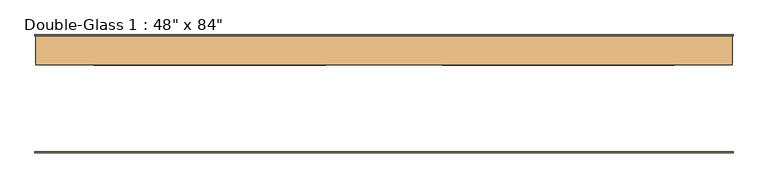
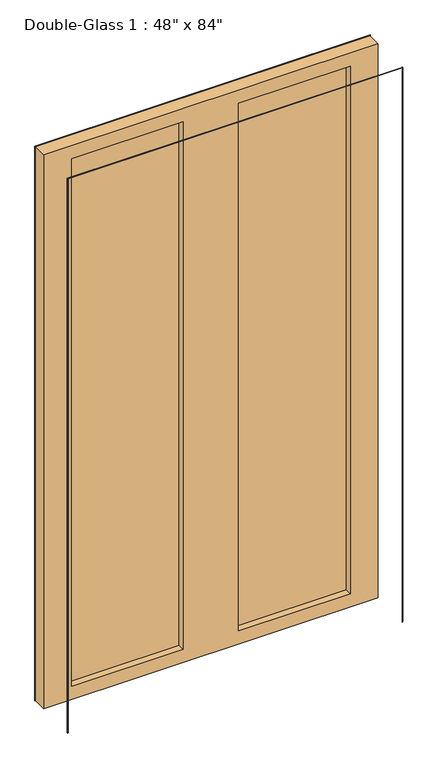
"""IFC4 building model written with IfcOpenShell, lengths in millimetres: door geometry."""

import ifcopenshell
import ifcopenshell.guid

model = None  # the IFC model being written
_history = None  # IfcOwnerHistory: only IFC2X3 demands one
_inside = {}  # id of a spatial element -> (the spatial element, [elements in it])
_under = {}  # id of a project, library or spatial element -> (it, [spatial elements below it])
_declared = {}  # id of a project -> (the project, [libraries it declares])
_typed = {}  # id of a type object -> (the type object, [elements of that type])
_made_of = {}  # id of a material, layer set ... -> (it, [elements and type objects made of it])


def new_model(schema):
    """Start an empty IFC model of exactly this schema.

    Asked for "IFC4X3", IfcOpenShell would pick the latest addendum, in which some entities
    have other attributes; the version numbers below select the first issue.
    IFC2X3 requires an IfcOwnerHistory on every rooted entity: one is made here for all.
    """
    global model, _history
    if schema == "IFC4X3":
        model = ifcopenshell.file(schema_version=(4, 3, 0, 0))
    else:
        model = ifcopenshell.file(schema=schema)
    _inside.clear()
    _under.clear()
    _declared.clear()
    _typed.clear()
    _made_of.clear()
    _history = None
    if model.schema == "IFC2X3":
        org = make("IfcOrganization", Name="unknown")
        user = make(
            "IfcPersonAndOrganization",
            ThePerson=make("IfcPerson", FamilyName="unknown"),
            TheOrganization=org,
        )
        app = make(
            "IfcApplication",
            ApplicationDeveloper=org,
            Version="unknown",
            ApplicationFullName="unknown",
            ApplicationIdentifier="unknown",
        )
        _history = make(
            "IfcOwnerHistory",
            OwningUser=user,
            OwningApplication=app,
            ChangeAction="ADDED",
            CreationDate=0,
        )
    return model


def make(cls, **values):
    """One entity of the class cls with the attributes given. An attribute that is None is left unset."""
    return model.create_entity(
        cls, **{name: value for name, value in values.items() if value is not None}
    )


def rooted(cls, **values):
    """An entity with a GlobalId (a new one), such as an element, a storey or a relation."""
    return make(cls, GlobalId=ifcopenshell.guid.new(), OwnerHistory=_history, **values)


def si_unit(unit_type, name, prefix=None):
    """IfcSIUnit, for example si_unit("LENGTHUNIT", "METRE", prefix="MILLI")."""
    return make("IfcSIUnit", UnitType=unit_type, Prefix=prefix, Name=name)


def assignment(units):
    """IfcUnitAssignment: the units of a project."""
    return None if units is None else make("IfcUnitAssignment", Units=units)


def point(xyz):
    """IfcCartesianPoint."""
    return None if xyz is None else make("IfcCartesianPoint", Coordinates=xyz)


def direction(xyz):
    """IfcDirection."""
    return None if xyz is None else make("IfcDirection", DirectionRatios=xyz)


def frame(location, z_axis=None, x_axis=None):
    """IfcAxis2Placement3D, a coordinate frame: its origin and axes. An axis left out is left unset."""
    return make(
        "IfcAxis2Placement3D",
        Location=point(location),
        Axis=direction(z_axis),
        RefDirection=direction(x_axis),
    )


def origin():
    """The frame at (0, 0, 0) with its axes left unset."""
    return frame((0.0, 0.0, 0.0))


def place(relative_to, where):
    """IfcLocalPlacement: puts the frame where relative to a parent placement (None: the world)."""
    return make(
        "IfcLocalPlacement", PlacementRelTo=relative_to, RelativePlacement=where
    )


def context(
    kind, dimensions, precision=None, world=None, true_north=None, identifier=None
):
    """IfcGeometricRepresentationContext, for example the 3D "Model" context."""
    return make(
        "IfcGeometricRepresentationContext",
        ContextIdentifier=identifier,
        ContextType=kind,
        CoordinateSpaceDimension=dimensions,
        Precision=precision,
        WorldCoordinateSystem=world,
        TrueNorth=true_north,
    )


def project(units=None, contexts=None):
    """IfcProject with its units and contexts."""
    return rooted(
        "IfcProject",
        Name="project",
        RepresentationContexts=contexts,
        UnitsInContext=assignment(units),
    )


def spatial(cls, under=None, at=None, **own):
    """A site, building, storey or space (cls), placed at a placement, below another one or the project."""
    s = rooted(cls, ObjectPlacement=at, **own)
    if under is not None:
        _under.setdefault(under.id(), (under, []))[1].append(s)
    return s


def polyline(points):
    """IfcPolyline through the points."""
    return make("IfcPolyline", Points=[point(p) for p in points])


def outline(outer, holes=None, kind="AREA"):
    """IfcArbitraryClosedProfileDef: a profile drawn as a closed curve; with holes, ...WithVoids."""
    if holes is None:
        return make("IfcArbitraryClosedProfileDef", ProfileType=kind, OuterCurve=outer)
    return make(
        "IfcArbitraryProfileDefWithVoids",
        ProfileType=kind,
        OuterCurve=outer,
        InnerCurves=holes,
    )


def extrude(swept, where, along, depth):
    """IfcExtrudedAreaSolid: the profile swept, set in the frame where, extruded along a direction by depth."""
    return make(
        "IfcExtrudedAreaSolid",
        SweptArea=swept,
        Position=where,
        ExtrudedDirection=direction(along),
        Depth=depth,
    )


def shape(context_of_items, identifier, shape_type, items):
    """IfcShapeRepresentation: the items that make up one representation, for example the "Body"."""
    return make(
        "IfcShapeRepresentation",
        ContextOfItems=context_of_items,
        RepresentationIdentifier=identifier,
        RepresentationType=shape_type,
        Items=items,
    )


def source(mapping_origin, context_of_items, identifier, shape_type, items):
    """IfcRepresentationMap: a shape defined once, which mapped items show again and again."""
    return make(
        "IfcRepresentationMap",
        MappingOrigin=mapping_origin,
        MappedRepresentation=shape(context_of_items, identifier, shape_type, items),
    )


def transform(
    local_origin,
    x_axis=None,
    y_axis=None,
    z_axis=None,
    scale=None,
    scale2=None,
    scale3=None,
    uniform=True,
):
    """IfcCartesianTransformationOperator3D, or its non-uniform kind. x_axis, y_axis, z_axis: its Axis1, 2, 3."""
    if uniform:
        return make(
            "IfcCartesianTransformationOperator3D",
            Axis1=direction(x_axis),
            Axis2=direction(y_axis),
            LocalOrigin=point(local_origin),
            Scale=scale,
            Axis3=direction(z_axis),
        )
    return make(
        "IfcCartesianTransformationOperator3DnonUniform",
        Axis1=direction(x_axis),
        Axis2=direction(y_axis),
        LocalOrigin=point(local_origin),
        Scale=scale,
        Axis3=direction(z_axis),
        Scale2=scale2,
        Scale3=scale3,
    )


def mapped(mapping_source, mapping_target):
    """IfcMappedItem: shows the shape of a source again, moved by a transform."""
    return make(
        "IfcMappedItem", MappingSource=mapping_source, MappingTarget=mapping_target
    )


def made_of(thing, what):
    """Note that an element or type object is made of a material, layer set ...; save() writes the relation."""
    if what is not None:
        _made_of.setdefault(what.id(), (what, []))[1].append(thing)
    return thing


def element(
    cls,
    number,
    at=None,
    inside=None,
    cuts=None,
    type_object=None,
    material=None,
    context=None,
    identifier="Body",
    shape_type=None,
    held_by="IfcProductDefinitionShape",
    body=None,
    shapes=None,
    **own,
):
    """One element of the class cls, such as IfcWall. Its Tag is "e" and its number.

    at: its placement. inside: the storey or other place that contains it. cuts: it is an
    opening in that element (IfcRelVoidsElement). A single representation is given by context,
    identifier, shape_type and body (its items); several are given by shapes. held_by: the class
    of the entity that holds the representations. save() writes the other relations.
    """
    e = rooted(cls, Tag="e%d" % number, ObjectPlacement=at, **own)
    if body is not None:
        shapes = [shape(context, identifier, shape_type, body)]
    if shapes is not None:
        e.Representation = make(held_by, Representations=shapes)
    if inside is not None:
        _inside.setdefault(inside.id(), (inside, []))[1].append(e)
    if cuts is not None:
        rooted(
            "IfcRelVoidsElement", RelatingBuildingElement=cuts, RelatedOpeningElement=e
        )
    if type_object is not None:
        _typed.setdefault(type_object.id(), (type_object, []))[1].append(e)
    return made_of(e, material)


def aggregate(whole, parts):
    """IfcRelAggregates: a whole, such as a stair, and the parts it consists of."""
    return rooted("IfcRelAggregates", RelatingObject=whole, RelatedObjects=parts)


def save(model, path):
    """Write the relations noted so far, then the file.

    IfcRelAggregates (storeys below a building ...), IfcRelContainedInSpatialStructure (elements
    in a storey), IfcRelDefinesByType, IfcRelAssociatesMaterial and IfcRelDeclares: one each for
    every whole, place, type object, material and project.
    """
    for whole, parts in _under.values():
        aggregate(whole, parts)
    for where, things in _inside.values():
        rooted(
            "IfcRelContainedInSpatialStructure",
            RelatedElements=things,
            RelatingStructure=where,
        )
    for kind, things in _typed.values():
        rooted("IfcRelDefinesByType", RelatedObjects=things, RelatingType=kind)
    for what, things in _made_of.values():
        rooted("IfcRelAssociatesMaterial", RelatedObjects=things, RelatingMaterial=what)
    for by, libraries in _declared.values():
        rooted("IfcRelDeclares", RelatingContext=by, RelatedDefinitions=libraries)
    model.write(path)


def door_f7b73743(model_context):
    return source(origin(), model_context, "Body", "SweptSolid", [
        extrude(outline(polyline([(0.0, 611.1875), (2135.1875, 611.1875), (2135.1875, -611.1875), (0.0, -611.1875), (0.0, -609.6), (2133.6, -609.6), (2133.6, 609.6), (0.0, 609.6), (0.0, 611.1875)])), frame((0.0, -100.80625, 0.0), z_axis=(0.0, 1.0, 0.0), x_axis=(0.0, 0.0, 1.0)), (0.0, 0.0, 1.0), 1.5875),
        extrude(outline(polyline([(2133.6, 609.6), (0.0, 609.6), (0.0, 611.1875), (2135.1875, 611.1875), (2135.1875, -611.1875), (0.0, -611.1875), (0.0, -609.6), (2133.6, -609.6), (2133.6, 609.6)])), frame((0.0, 103.98125, 0.0), z_axis=(0.0, 1.0, 0.0), x_axis=(0.0, 0.0, 1.0)), (0.0, 0.0, 1.0), 1.5875),
        extrude(outline(polyline([(508.0, 78.58125), (101.6, 78.58125), (101.6, 85.725), (508.0, 85.725), (508.0, 78.58125)])), frame((0.0, 0.0, 50.8), z_axis=(0.0, 0.0, 1.0), x_axis=(1.0, 0.0, 0.0)), (0.0, 0.0, 1.0), 2032.0),
        extrude(outline(polyline([(-101.6, 78.58125), (-508.0, 78.58125), (-508.0, 85.725), (-101.6, 85.725), (-101.6, 78.58125)])), frame((0.0, 0.0, 50.8), z_axis=(0.0, 0.0, 1.0), x_axis=(1.0, 0.0, 0.0)), (0.0, 0.0, 1.0), 2032.0),
        extrude(outline(polyline([(2133.6, 609.6), (2133.6, -609.6), (0.0, -609.6), (0.0, 609.6), (2133.6, 609.6)]), holes=[polyline([(2082.8, -101.6), (50.8, -101.6), (50.8, -508.0), (2082.8, -508.0), (2082.8, -101.6)]), polyline([(2082.8, 508.0), (50.8, 508.0), (50.8, 101.6), (2082.8, 101.6), (2082.8, 508.0)])]), frame((0.0, 53.18125, 0.0), z_axis=(0.0, 1.0, 0.0), x_axis=(0.0, 0.0, 1.0)), (0.0, 0.0, 1.0), 50.8),
    ])


if __name__ == "__main__":
    model = new_model("IFC4")
    model_context = context("Model", 3, world=origin())
    ifc_project = project(units=[si_unit("LENGTHUNIT", "METRE", prefix="MILLI")], contexts=[model_context])
    site = spatial("IfcSite", under=ifc_project)
    building = spatial("IfcBuilding", under=site)
    placement = place(None, origin())
    door_shape = door_f7b73743(model_context)
    element("IfcDoor", 1, ObjectType="Double-Glass 1 : 48\" x 84\"", at=placement, inside=building, context=model_context, shape_type="MappedRepresentation", body=[
        mapped(door_shape, transform((0.0, 0.0, 0.0), x_axis=(1.0, 0.0, 0.0), y_axis=(0.0, 1.0, 0.0), z_axis=(0.0, 0.0, 1.0))),
    ])
    save(model, "model.ifc")

# Revit data of these elements
# Type "Double-Glass 1 : 48\" x 84\""
#   Type Mark = "21"
#   Assembly Code = "C1020"
#   Thickness = 50.80 mm
#   Height = 2133.60 mm
#   Rail Width - Base = 50.80 mm
#   Rail Width - Top = 50.80 mm
#   Stile Width - Hinge = 50.80 mm
#   Stile Width - Latch = 50.80 mm
#   Trim Projection = 1.587 mm
#   Trim Width = 1.587 mm
#   Width = 1219.20 mm
#   Door Material = Door - Panel
#   Frame Material = Door - Frame
#   Function = (empty or 0)
#   Wall Closure = (empty or 0)
# Element 1 (IfcDoor, "Double-Glass 1 : 48\" x 84\"")
#   Materials on its faces: "Door - Frame", "Door - Panel", "Glass"
# Materials
#   "Door - Panel": class "Wood", colour RGB 210 159 95, transparency 0
#   "Door - Frame": class "Miscellaneous", colour RGB 118 70 51, transparency 0
#   "Glass": class "Glass", colour RGB 0 128 192, transparency 0.75
